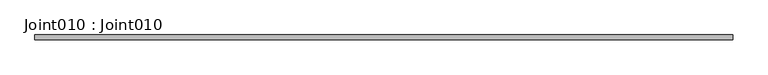
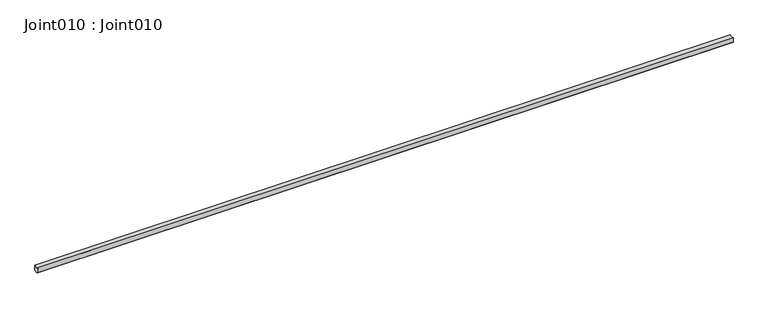
"""IFC4 building model written with IfcOpenShell, lengths in millimetres: proxy geometry, Joint010 : Joint010."""

from ifc_helpers import new_model, si_unit, point, frame, frame_2d, origin, place, context, project, spatial, polyline, circle_curve, trimmed, segment, composite_curve, outline, extrude, source, transform, mapped, element, save


def joint010_joint010_dbf7cb60(model_context):
    return source(origin(), model_context, "Body", "SweptSolid", [
        extrude(outline(composite_curve([segment(trimmed(circle_curve(frame_2d((-4644.5231449, 36335.014173)), 9.8285468), [point((-4651.5044925, 36328.096))], [point((-4637.5417972, 36328.096))], True, "CARTESIAN"), True, "CONTINUOUS"), segment(polyline([(-4637.5417972, 36328.096), (-4637.5417972, 36313.846)]), True, "CONTINUOUS"), segment(trimmed(circle_curve(frame_2d((-4644.5231449, 36320.764173)), 9.8285468), [point((-4637.5417972, 36313.846))], [point((-4651.5044925, 36313.846))], False, "CARTESIAN"), True, "CONTINUOUS"), segment(polyline([(-4651.5044925, 36313.846), (-4651.5044925, 36328.096)]), True, "CONTINUOUS")], self_intersect=False)), frame((12383.0178845, 0.0, 0.0), z_axis=(1.0, 0.0, 0.0), x_axis=(0.0, 1.0, 0.0)), (0.0, 0.0, 1.0), 2000.0),
    ])


if __name__ == "__main__":
    model = new_model("IFC4")
    model_context = context("Model", 3, world=origin())
    ifc_project = project(units=[si_unit("LENGTHUNIT", "METRE", prefix="MILLI")], contexts=[model_context])
    site = spatial("IfcSite", under=ifc_project)
    building = spatial("IfcBuilding", under=site)
    placement = place(None, origin())
    joint010_joint010_shape = joint010_joint010_dbf7cb60(model_context)
    element("IfcBuildingElementProxy", 1, Name="Joint010 : Joint010", ObjectType="Joint010 : Joint010", at=placement, inside=building, context=model_context, shape_type="MappedRepresentation", body=[
        mapped(joint010_joint010_shape, transform((0.0, 0.0, 0.0), x_axis=(1.0, 0.0, 0.0), y_axis=(0.0, 1.0, 0.0), z_axis=(0.0, 0.0, 1.0))),
    ])
    save(model, "model.ifc")

# Revit data of these elements
# Type "Joint010 : Joint010"
#   NameOverride = "Joint010"
# Element 1 (IfcBuildingElementProxy, "Joint010 : Joint010")
#   Materials on its faces: "SEALANT JOINT"
# Materials
#   "SEALANT JOINT": class "Unassigned", colour RGB 142 225 148, transparency 0
